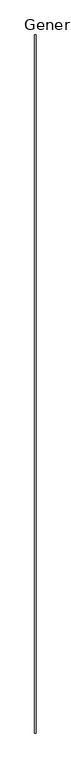
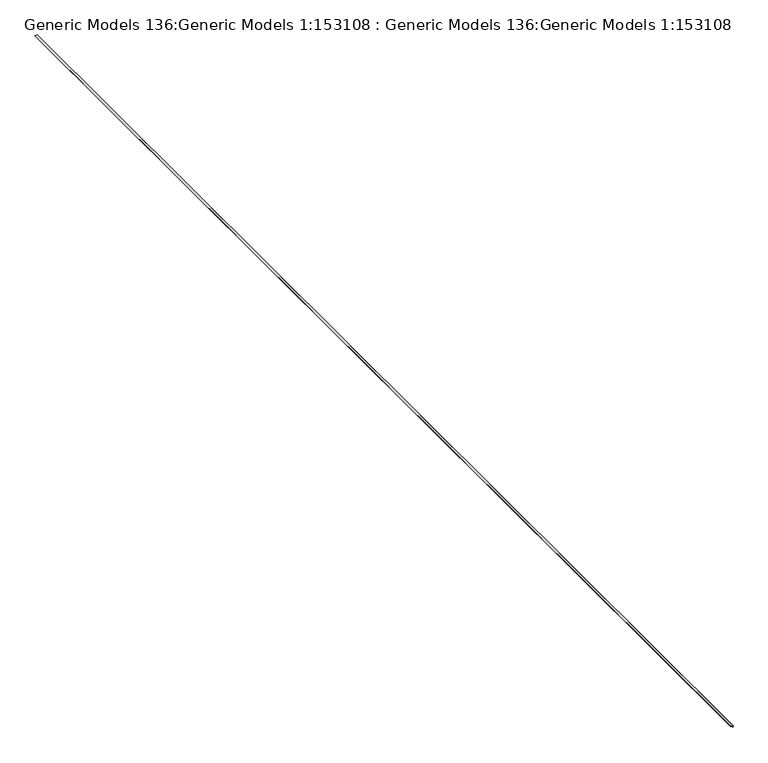
"""IFC4 building model written with IfcOpenShell, lengths in millimetres: proxy geometry, Generic Models 136:Generic Models 1:153108 : Generic Models 136:Generic Models 1:153108."""

from ifc_helpers import new_model, si_unit, frame, origin, place, context, project, spatial, polyline, outline, extrude, source, transform, mapped, element, save


def generic_models_136_generic_models_1_153108_generic_models_6c538806(model_context):
    return source(origin(), model_context, "Body", "SweptSolid", [
        extrude(outline(polyline([(3044.825, 7231.429663), (3044.825, 7236.179463), (3067.05, 7236.179463), (3067.05, 7198.079463), (3065.78, 7198.079463), (3065.78, 7234.909463), (3046.095, 7234.909463), (3046.095, 7232.699663), (3047.8274564, 7232.699663), (3047.8274564, 7231.429663), (3044.825, 7231.429663)])), frame((0.0, -6877.9974793, 0.0), z_axis=(0.0, 1.0, 0.0), x_axis=(0.0, 0.0, 1.0)), (0.0, 0.0, 1.0), 19050.0),
    ])


if __name__ == "__main__":
    model = new_model("IFC4")
    model_context = context("Model", 3, world=origin())
    ifc_project = project(units=[si_unit("LENGTHUNIT", "METRE", prefix="MILLI")], contexts=[model_context])
    site = spatial("IfcSite", under=ifc_project)
    building = spatial("IfcBuilding", under=site)
    placement = place(None, origin())
    generic_models_136_generic_models_1_153108_generic_models_shape = generic_models_136_generic_models_1_153108_generic_models_6c538806(model_context)
    element("IfcBuildingElementProxy", 1, Name="Generic Models 136:Generic Models 1:153108 : Generic Models 136:Generic Models 1:153108", ObjectType="Generic Models 136:Generic Models 1:153108 : Generic Models 136:Generic Models 1:153108", at=placement, inside=building, context=model_context, shape_type="MappedRepresentation", body=[
        mapped(generic_models_136_generic_models_1_153108_generic_models_shape, transform((0.0, 0.0, 0.0), x_axis=(1.0, 0.0, 0.0), y_axis=(0.0, 1.0, 0.0), z_axis=(0.0, 0.0, 1.0))),
    ])
    save(model, "model.ifc")

# Revit data of these elements
# Type "Generic Models 136:Generic Models 1:153108 : Generic Models 136:Generic Models 1:153108"
#   NameOverride = "Generic Models 136:Generic Models 1:153108"
#   ObjectTypeOverride = "Generic Models 136:Generic Models 1"
#   Reference = "Generic Models 1"
#   Category = "Generic Models"
#   Tag = "153108"
# Element 1 (IfcBuildingElementProxy, "Generic Models 136:Generic Models 1:153108 : Generic Models 136:Generic Models 1:153108")
#   Materials on its faces: "_CONTINUOUS 16 GA. COPPER  J BEAD 1960"
# Materials
#   "_CONTINUOUS 16 GA. COPPER  J BEAD 1960": class "Unassigned", colour RGB 253 192 103, transparency 0
